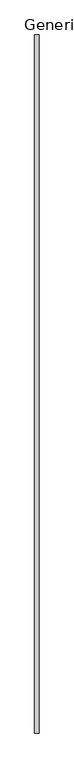
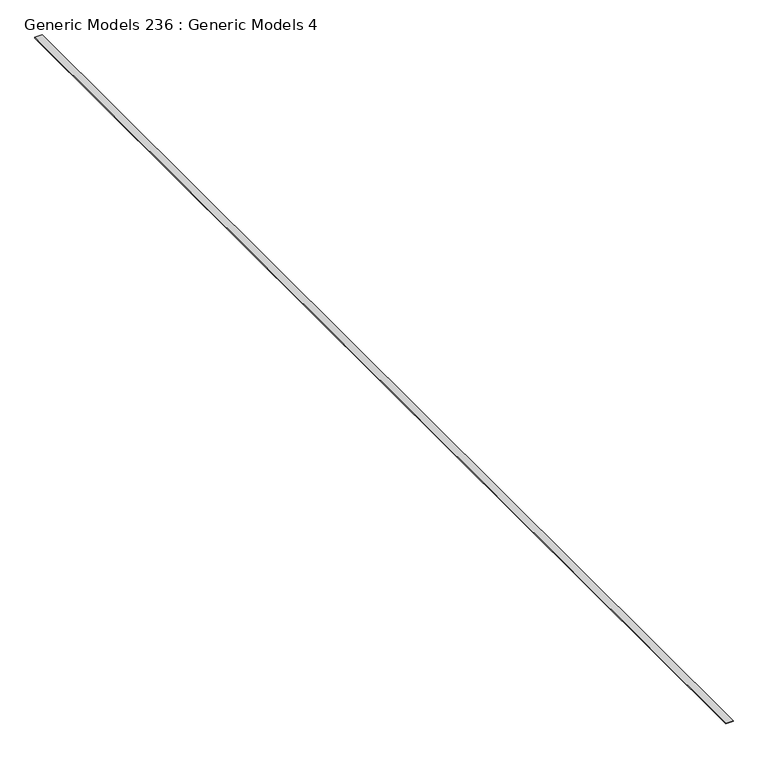
"""IFC4 building model written with IfcOpenShell, lengths in millimetres: proxy geometry, Generic Models 236 : Generic Models 4."""

from ifc_helpers import new_model, si_unit, frame, origin, place, context, project, spatial, polyline, outline, extrude, source, transform, mapped, element, save


def generic_models_236_generic_models_4_2946484d(model_context):
    return source(origin(), model_context, "Body", "SweptSolid", [
        extrude(outline(polyline([(35688.6626306, 12775.6158826), (35776.3520399, 12775.6158826), (35776.3520399, -1143.5841174), (35688.6626306, -1143.5841174), (35688.6626306, 12775.6158826)])), frame((0.0, 0.0, 129263.3128468), z_axis=(0.0, 0.0, 1.0), x_axis=(1.0, 0.0, 0.0)), (0.0, 0.0, 1.0), 9.525),
    ])


if __name__ == "__main__":
    model = new_model("IFC4")
    model_context = context("Model", 3, world=origin())
    ifc_project = project(units=[si_unit("LENGTHUNIT", "METRE", prefix="MILLI")], contexts=[model_context])
    site = spatial("IfcSite", under=ifc_project)
    building = spatial("IfcBuilding", under=site)
    placement = place(None, origin())
    generic_models_236_generic_models_4_shape = generic_models_236_generic_models_4_2946484d(model_context)
    element("IfcBuildingElementProxy", 1, Name="Generic Models 236 : Generic Models 4", ObjectType="Generic Models 236 : Generic Models 4", at=placement, inside=building, context=model_context, shape_type="MappedRepresentation", body=[
        mapped(generic_models_236_generic_models_4_shape, transform((0.0, 0.0, 0.0), x_axis=(1.0, 0.0, 0.0), y_axis=(0.0, 1.0, 0.0), z_axis=(0.0, 0.0, 1.0))),
    ])
    save(model, "model.ifc")

# Revit data of these elements
# Element 1 (IfcBuildingElementProxy, "Generic Models 236 : Generic Models 4")
#   Materials on its faces: "_BLOCKING AS REQUIRED"
# Materials
#   "_BLOCKING AS REQUIRED": class "Generic", colour RGB 177 130 114, transparency 0, Cost = 0
